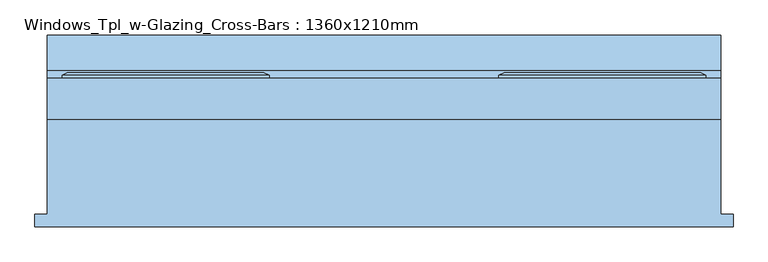
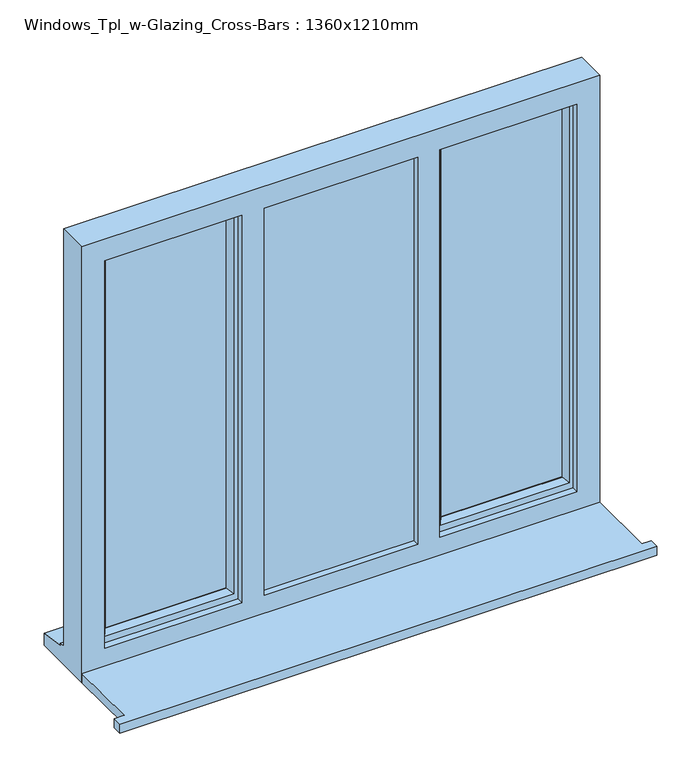
"""IFC4 building model written with IfcOpenShell, lengths in millimetres: window geometry, Windows_Tpl_w-Glazing_Cross-Bars : 1360x1210mm."""

from ifc_helpers import new_model, si_unit, frame, origin, place, context, project, spatial, polyline, outline, extrude, faceted_brep, source, transform, mapped, element, save


def windows_tpl_w_glazing_cross_bars_1360x1210mm_fa1f7dc8(model_context):
    return source(origin(), model_context, "Body", "SolidModel", [
        extrude(outline(polyline([(-1206.6666667, -178.7934322), (-1206.6666667, -153.7934322), (-1181.6666667, -153.7934322), (-1181.6666667, 37.7065678), (178.3333333, 37.7065678), (178.3333333, -153.7934322), (203.3333333, -153.7934322), (203.3333333, -178.7934322), (-1206.6666667, -178.7934322)])), frame((0.0, 0.0, 900.0), z_axis=(0.0, 0.0, 1.0), x_axis=(1.0, 0.0, 0.0)), (0.0, 0.0, 1.0), 25.0),
        extrude(outline(polyline([(-773.3333333, 72.4565678), (-1111.6666667, 72.4565678), (-1111.6666667, 96.4565678), (-773.3333333, 96.4565678), (-773.3333333, 72.4565678)])), frame((0.0, 0.0, 993.0), z_axis=(0.0, 0.0, 1.0), x_axis=(1.0, 0.0, 0.0)), (0.0, 0.0, 1.0), 1047.0),
        extrude(outline(polyline([(108.4813711, 72.4565678), (-230.1480377, 72.4565678), (-230.1480377, 96.4565678), (108.4813711, 96.4565678), (108.4813711, 72.4565678)])), frame((0.0, 0.0, 992.8519623), z_axis=(0.0, 0.0, 1.0), x_axis=(1.0, 0.0, 0.0)), (0.0, 0.0, 1.0), 1047.2960754),
        extrude(outline(polyline([(-713.3333333, 79.7065678), (-290.0, 79.7065678), (-290.0, 55.7065678), (-713.3333333, 55.7065678), (-713.3333333, 79.7065678)])), frame((0.0, 0.0, 963.0), z_axis=(0.0, 0.0, 1.0), x_axis=(1.0, 0.0, 0.0)), (0.0, 0.0, 1.0), 1107.0),
        faceted_brep([(178.3333333, 37.7065678, 2110.0), (-1181.6666667, 37.7065678, 2110.0), (-1181.6666667, 37.7065678, 900.0), (178.3333333, 37.7065678, 900.0), (118.3333333, 37.7065678, 2050.0), (118.3333333, 37.7065678, 975.0), (-242.0, 37.7065678, 975.0), (-242.0, 37.7065678, 2050.0), (-300.0, 37.7065678, 2050.0), (-300.0, 37.7065678, 975.0), (-703.3333333, 37.7065678, 975.0), (-703.3333333, 37.7065678, 2050.0), (-761.3333333, 37.7065678, 2050.0), (-761.3333333, 37.7065678, 975.0), (-1121.6666667, 37.7065678, 975.0), (-1121.6666667, 37.7065678, 2050.0), (-1181.6666667, 120.7065678, 2110.0), (-1181.6666667, 120.7065678, 951.0), (-1181.6666667, 135.7065678, 949.68767), (-1181.6666667, 135.7065678, 944.7449676), (-1181.6666667, 208.2065678, 933.8088847), (-1181.6666667, 208.2065678, 900.0), (178.3333333, 120.7065678, 2110.0), (178.3333333, 120.7065678, 951.0), (-1141.6666667, 120.7065678, 2070.0), (-1141.6666667, 120.7065678, 963.0), (-743.3333333, 120.7065678, 963.0), (-743.3333333, 120.7065678, 2070.0), (-703.3333333, 120.7065678, 2070.0), (-703.3333333, 120.7065678, 963.0), (-300.0, 120.7065678, 963.0), (-300.0, 120.7065678, 2070.0), (-260.0, 120.7065678, 2070.0), (-260.0, 120.7065678, 963.0), (138.3333333, 120.7065678, 963.0), (138.3333333, 120.7065678, 2070.0), (-1141.6666667, 55.7065678, 2070.0), (-1141.6666667, 55.7065678, 963.0), (-713.3333333, 55.7065678, 2070.0), (-290.0, 55.7065678, 2070.0), (-290.0, 55.7065678, 963.0), (-713.3333333, 55.7065678, 963.0), (-300.0, 55.7065678, 2050.0), (-703.3333333, 55.7065678, 2050.0), (-703.3333333, 55.7065678, 975.0), (-300.0, 55.7065678, 975.0), (-260.0, 55.7065678, 2070.0), (138.3333333, 55.7065678, 2070.0), (138.3333333, 55.7065678, 963.0), (-260.0, 55.7065678, 963.0), (118.3333333, 55.7065678, 2050.0), (-242.0, 55.7065678, 2050.0), (-242.0, 55.7065678, 975.0), (118.3333333, 55.7065678, 975.0), (-743.3333333, 55.7065678, 2070.0), (-743.3333333, 55.7065678, 963.0), (-761.3333333, 55.7065678, 2050.0), (-1121.6666667, 55.7065678, 2050.0), (-1121.6666667, 55.7065678, 975.0), (-761.3333333, 55.7065678, 975.0), (-703.3333333, 79.7065678, 2070.0), (-300.0, 79.7065678, 2070.0), (-290.0, 79.7065678, 2070.0), (-713.3333333, 79.7065678, 2070.0), (178.3333333, 208.2065678, 900.0), (178.3333333, 208.2065678, 933.8088847), (178.3333333, 135.7065678, 944.7449676), (178.3333333, 135.7065678, 949.68767), (-703.3333333, 79.7065678, 963.0), (-713.3333333, 79.7065678, 963.0), (-290.0, 79.7065678, 963.0), (-300.0, 79.7065678, 963.0)], [[[0, 1, 2, 3], [4, 5, 6, 7], [8, 9, 10, 11], [12, 13, 14, 15]], [[2, 1, 16, 17, 18, 19, 20, 21]], [[17, 16, 22, 23], [24, 25, 26, 27], [28, 29, 30, 31], [32, 33, 34, 35]], [[25, 24, 36, 37]], [[38, 39, 40, 41], [42, 43, 44, 45]], [[46, 47, 48, 49], [50, 51, 52, 53]], [[36, 54, 55, 37], [56, 57, 58, 59]], [[57, 15, 14, 58]], [[1, 0, 22, 16]], [[36, 24, 27, 54]], [[35, 47, 46, 32]], [[60, 28, 31, 61, 62, 39, 38, 63]], [[15, 57, 56, 12]], [[50, 4, 7, 51]], [[11, 43, 42, 8]], [[23, 22, 0, 3, 64, 65, 66, 67]], [[35, 34, 48, 47]], [[4, 50, 53, 5]], [[43, 11, 10, 44]], [[12, 56, 59, 13]], [[27, 26, 55, 54]], [[29, 28, 60, 68]], [[68, 60, 63, 69]], [[69, 63, 38, 41]], [[62, 70, 40, 39]], [[70, 62, 61, 71]], [[71, 61, 31, 30]], [[33, 32, 46, 49]], [[51, 7, 6, 52]], [[8, 42, 45, 9]], [[64, 3, 2, 21]], [[65, 64, 21, 20]], [[66, 65, 20, 19]], [[67, 66, 19, 18]], [[23, 67, 18, 17]], [[26, 25, 37, 55]], [[34, 33, 49, 48]], [[41, 40, 70, 71, 30, 29, 68, 69]], [[6, 5, 53, 52]], [[45, 44, 10, 9]], [[59, 58, 14, 13]]]),
        extrude(outline(polyline([(963.0, -511.6666667), (963.0, -491.6666667), (1506.5, -491.6666667), (1506.5, -290.0), (1526.5, -290.0), (1526.5, -491.6666667), (2070.0, -491.6666667), (2070.0, -511.6666667), (1526.5, -511.6666667), (1526.5, -713.3333333), (1506.5, -713.3333333), (1506.5, -511.6666667), (963.0, -511.6666667)])), frame((0.0, 63.7065678, 0.0), z_axis=(0.0, 1.0, 0.0), x_axis=(0.0, 0.0, 1.0)), (0.0, 0.0, 1.0), 8.0),
        extrude(outline(polyline([(993.0, -70.8333333), (993.0, -50.8333333), (1506.5, -50.8333333), (1506.5, 108.3333333), (1526.5, 108.3333333), (1526.5, -50.8333333), (2040.1480377, -50.8333333), (2040.1480377, -70.8333333), (1526.5, -70.8333333), (1526.5, -230.1480377), (1506.5, -230.1480377), (1506.5, -70.8333333), (993.0, -70.8333333)])), frame((0.0, 92.7065678, 0.0), z_axis=(0.0, 1.0, 0.0), x_axis=(0.0, 0.0, 1.0)), (0.0, 0.0, 1.0), 8.0),
        extrude(outline(polyline([(993.0, -952.5), (993.0, -932.5), (1506.5, -932.5), (1506.5, -773.3333333), (1526.5, -773.3333333), (1526.5, -932.5), (2040.1480377, -932.5), (2040.1480377, -952.5), (1526.5, -952.5), (1526.5, -1111.6666667), (1506.5, -1111.6666667), (1506.5, -952.5), (993.0, -952.5)])), frame((0.0, 92.7065678, 0.0), z_axis=(0.0, 1.0, 0.0), x_axis=(0.0, 0.0, 1.0)), (0.0, 0.0, 1.0), 8.0),
        faceted_brep([(-733.3333333, 120.7065678, 2080.0), (-733.3333333, 126.4800705, 2080.0), (-1151.6666667, 126.4800705, 2080.0), (-1151.6666667, 120.7065678, 2080.0), (-743.3333333, 55.7065678, 2070.0), (-743.3333333, 120.7065678, 2070.0), (-1141.6666667, 120.7065678, 2070.0), (-1141.6666667, 55.7065678, 2070.0), (-783.3333333, 70.1994677, 2030.0), (-773.1852956, 55.7065678, 2040.1480377), (-1111.8147044, 55.7065678, 2040.1480377), (-1101.6666667, 70.1994677, 2030.0), (-783.3333333, 84.7065678, 2030.0), (-1101.6666667, 84.7065678, 2030.0), (-773.3333333, 108.7065678, 2040.0), (-773.3333333, 84.7065678, 2040.0), (-1111.6666667, 84.7065678, 2040.0), (-1111.6666667, 108.7065678, 2040.0), (-783.3333333, 126.4800705, 2030.0), (-783.3333333, 108.7065678, 2030.0), (-1101.6666667, 108.7065678, 2030.0), (-1101.6666667, 126.4800705, 2030.0), (-765.8875785, 132.2535732, 2047.4457548), (-1119.1124215, 132.2535732, 2047.4457548), (-744.117943, 132.2535732, 2069.2153903), (-1140.882057, 132.2535732, 2069.2153903), (-1151.6666667, 126.4800705, 953.0), (-1151.6666667, 120.7065678, 953.0), (-1141.6666667, 120.7065678, 963.0), (-1141.6666667, 55.7065678, 963.0), (-1111.8147044, 55.7065678, 992.8519623), (-1101.6666667, 70.1994677, 1003.0), (-1101.6666667, 84.7065678, 1003.0), (-1111.6666667, 84.7065678, 993.0), (-1111.6666667, 108.7065678, 993.0), (-1101.6666667, 108.7065678, 1003.0), (-1101.6666667, 126.4800705, 1003.0), (-1119.1124215, 132.2535732, 985.5542452), (-1140.882057, 132.2535732, 963.7846097), (-733.3333333, 126.4800705, 953.0), (-733.3333333, 120.7065678, 953.0), (-743.3333333, 120.7065678, 963.0), (-743.3333333, 55.7065678, 963.0), (-773.1852956, 55.7065678, 992.8519623), (-783.3333333, 70.1994677, 1003.0), (-783.3333333, 84.7065678, 1003.0), (-773.3333333, 84.7065678, 993.0), (-773.3333333, 108.7065678, 993.0), (-783.3333333, 108.7065678, 1003.0), (-783.3333333, 126.4800705, 1003.0), (-765.8875785, 132.2535732, 985.5542452), (-744.117943, 132.2535732, 963.7846097)], [[[0, 1, 2, 3]], [[4, 5, 6, 7]], [[8, 9, 10, 11]], [[12, 8, 11, 13]], [[14, 15, 16, 17]], [[18, 19, 20, 21]], [[22, 18, 21, 23]], [[1, 24, 25, 2]], [[3, 2, 26, 27]], [[7, 6, 28, 29]], [[11, 10, 30, 31]], [[13, 11, 31, 32]], [[17, 16, 33, 34]], [[21, 20, 35, 36]], [[23, 21, 36, 37]], [[2, 25, 38, 26]], [[27, 26, 39, 40]], [[0, 3, 27, 40], [41, 28, 6, 5]], [[29, 28, 41, 42]], [[4, 7, 29, 42], [43, 30, 10, 9]], [[31, 30, 43, 44]], [[32, 31, 44, 45]], [[46, 33, 16, 15], [12, 13, 32, 45]], [[34, 33, 46, 47]], [[14, 17, 34, 47], [48, 35, 20, 19]], [[36, 35, 48, 49]], [[37, 36, 49, 50]], [[51, 38, 25, 24], [22, 23, 37, 50]], [[26, 38, 51, 39]], [[40, 39, 1, 0]], [[42, 41, 5, 4]], [[44, 43, 9, 8]], [[45, 44, 8, 12]], [[47, 46, 15, 14]], [[49, 48, 19, 18]], [[50, 49, 18, 22]], [[39, 51, 24, 1]]]),
        faceted_brep([(-270.0, 120.7065678, 2080.0), (-270.0, 126.4800705, 2080.0), (-270.0, 126.4800705, 953.0), (-270.0, 120.7065678, 953.0), (-260.0, 55.7065678, 2070.0), (-260.0, 120.7065678, 2070.0), (-260.0, 120.7065678, 963.0), (-260.0, 55.7065678, 963.0), (-220.0, 70.1994677, 2030.0), (-230.1480377, 55.7065678, 2040.1480377), (-230.1480377, 55.7065678, 992.8519623), (-220.0, 70.1994677, 1003.0), (-220.0, 84.7065678, 2030.0), (-220.0, 84.7065678, 1003.0), (-230.0, 108.7065678, 2040.0), (-230.0, 84.7065678, 2040.0), (-230.0, 84.7065678, 993.0), (-230.0, 108.7065678, 993.0), (-220.0, 126.4800705, 2030.0), (-220.0, 108.7065678, 2030.0), (-220.0, 108.7065678, 1003.0), (-220.0, 126.4800705, 1003.0), (-237.4457548, 132.2535732, 2047.4457548), (-237.4457548, 132.2535732, 985.5542452), (-259.2153903, 132.2535732, 2069.2153903), (-259.2153903, 132.2535732, 963.7846097), (148.3333333, 126.4800705, 953.0), (148.3333333, 120.7065678, 953.0), (138.3333333, 120.7065678, 963.0), (138.3333333, 55.7065678, 963.0), (108.4813711, 55.7065678, 992.8519623), (98.3333333, 70.1994677, 1003.0), (98.3333333, 84.7065678, 1003.0), (108.3333333, 84.7065678, 993.0), (108.3333333, 108.7065678, 993.0), (98.3333333, 108.7065678, 1003.0), (98.3333333, 126.4800705, 1003.0), (115.7790881, 132.2535732, 985.5542452), (137.5487236, 132.2535732, 963.7846097), (148.3333333, 126.4800705, 2080.0), (148.3333333, 120.7065678, 2080.0), (138.3333333, 120.7065678, 2070.0), (138.3333333, 55.7065678, 2070.0), (108.4813711, 55.7065678, 2040.1480377), (98.3333333, 70.1994677, 2030.0), (98.3333333, 84.7065678, 2030.0), (108.3333333, 84.7065678, 2040.0), (108.3333333, 108.7065678, 2040.0), (98.3333333, 108.7065678, 2030.0), (98.3333333, 126.4800705, 2030.0), (115.7790881, 132.2535732, 2047.4457548), (137.5487236, 132.2535732, 2069.2153903)], [[[0, 1, 2, 3]], [[4, 5, 6, 7]], [[8, 9, 10, 11]], [[12, 8, 11, 13]], [[14, 15, 16, 17]], [[18, 19, 20, 21]], [[22, 18, 21, 23]], [[1, 24, 25, 2]], [[3, 2, 26, 27]], [[7, 6, 28, 29]], [[11, 10, 30, 31]], [[13, 11, 31, 32]], [[17, 16, 33, 34]], [[21, 20, 35, 36]], [[23, 21, 36, 37]], [[2, 25, 38, 26]], [[27, 26, 39, 40]], [[29, 28, 41, 42]], [[31, 30, 43, 44]], [[32, 31, 44, 45]], [[34, 33, 46, 47]], [[36, 35, 48, 49]], [[37, 36, 49, 50]], [[26, 38, 51, 39]], [[40, 39, 1, 0]], [[3, 27, 40, 0], [5, 41, 28, 6]], [[42, 41, 5, 4]], [[7, 29, 42, 4], [9, 43, 30, 10]], [[44, 43, 9, 8]], [[45, 44, 8, 12]], [[15, 46, 33, 16], [13, 32, 45, 12]], [[47, 46, 15, 14]], [[17, 34, 47, 14], [19, 48, 35, 20]], [[49, 48, 19, 18]], [[50, 49, 18, 22]], [[24, 51, 38, 25], [23, 37, 50, 22]], [[39, 51, 24, 1]]]),
    ])


if __name__ == "__main__":
    model = new_model("IFC4")
    model_context = context("Model", 3, world=origin())
    ifc_project = project(units=[si_unit("LENGTHUNIT", "METRE", prefix="MILLI")], contexts=[model_context])
    site = spatial("IfcSite", under=ifc_project)
    building = spatial("IfcBuilding", under=site)
    placement = place(None, origin())
    windows_tpl_w_glazing_cross_bars_1360x1210mm_shape = windows_tpl_w_glazing_cross_bars_1360x1210mm_fa1f7dc8(model_context)
    element("IfcWindow", 1, ObjectType="Windows_Tpl_w-Glazing_Cross-Bars : 1360x1210mm", at=placement, inside=building, context=model_context, shape_type="MappedRepresentation", body=[
        mapped(windows_tpl_w_glazing_cross_bars_1360x1210mm_shape, transform((0.0, 0.0, 0.0), x_axis=(1.0, 0.0, 0.0), y_axis=(0.0, 1.0, 0.0), z_axis=(0.0, 0.0, 1.0))),
    ])
    save(model, "model.ifc")

# Revit data of these elements
# Type "Windows_Tpl_w-Glazing_Cross-Bars : 1360x1210mm"
#   Type Mark = "53"
#   Operation = "TriplePanelVertical"
#   Construction Type Id = "GSP4R"
#   Manufacturer = "Revit"
#   Keynote = "L10"
#   Analytic Construction = "1/8 in Pilkington single glazing"
#   Wrap Layers (Ext) from Ext = 102.5 mm
#   Wrap Layers (Int) from Ext = 177.5 mm
#   Window Board Projection = 25 mm
#   Window Board Extension = 25 mm
#   Visual Light Transmittance = 0.9
#   Solar Heat Gain Coefficient = 0.78
#   Rough Width = 1360 mm
#   Rough Height = 1210 mm
#   Height = 1210 mm
#   Width = 1360 mm
#   Heat Transfer Coefficient (U) = 3.6886 W/(m²·K)
#   Glazing Thickness = 24 mm
#   Glazing Bar Thickness = 20 mm
#   FrameOffset - External = 50 mm
#   Frame Depth = 65 mm
#   Default Head Height = 2110 mm
#   Cill Depth = 87.5 mm
#   Cavity Closer Width = 50 mm
#   Cavity Closer Offset from Ext = 102.5 mm
#   Cavity Closer Depth = 85 mm
#   Vis - Glazing Bars = yes
#   Vis - Cavity Closers = yes
#   Material Trim = Window Frame
#   Material Glazing Bars = Window Frame
#   Material Glass = Glass
#   Material Frame = Window Frame
#   Wall Closure = (empty or 0)
# Element 1 (IfcWindow, "Windows_Tpl_w-Glazing_Cross-Bars : 1360x1210mm")
#   Materials on its faces: "Window Frame", "Glass"
# Materials
#   "Window Frame": class "Miscellaneous", colour RGB 249 249 249, transparency 0, Keynote = "L10"
#   "Glass": class "Glass", colour RGB 0 128 192, transparency 0.9, Description = "Soda Lime Glass", Cost = 0
